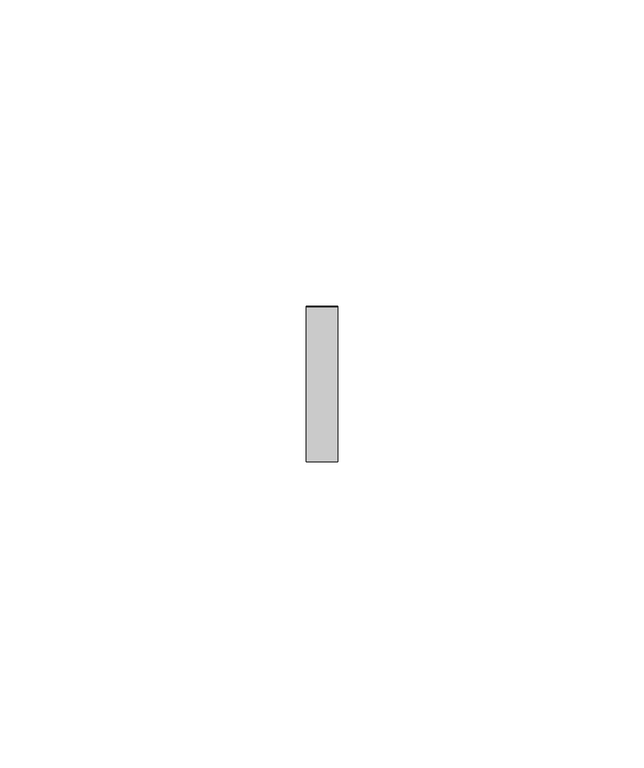
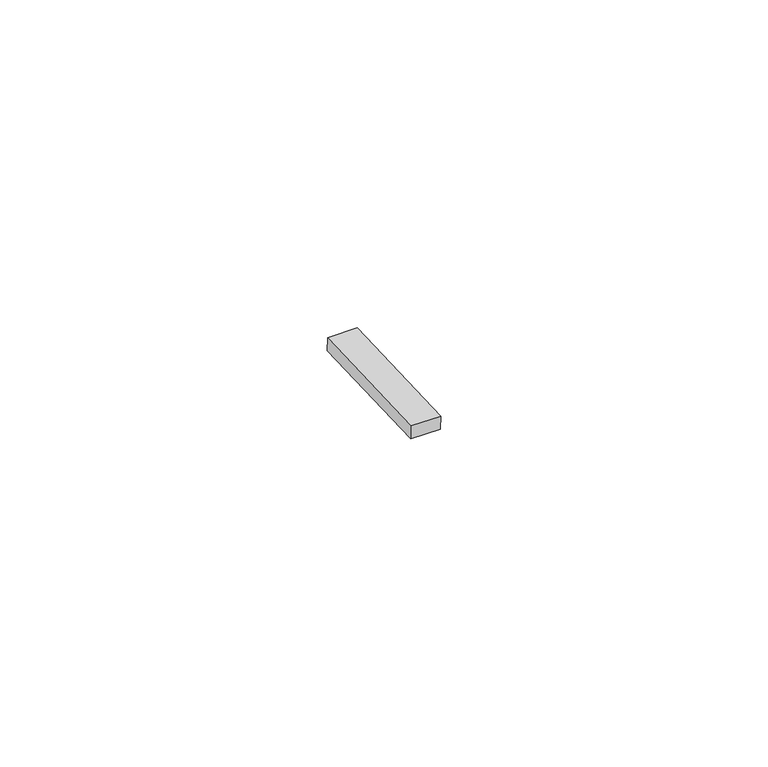
"""IFC4 building model written with IfcOpenShell, lengths in millimetres: proxy geometry, Inner panel:Inner panel:1:Inner panel:1 : Inner panel:Inner panel:300324:2:Inner panel:1:Inner panel:1 : Inner panel:Inner panel:300324:2 : Inner panel:Inner panel:1:Inner panel:1 : Inner panel:Inner panel:300324:300043:111 : Inner panel:Inner panel:1:Inner panel:1 : Inner panel:Inner panel:300324:2:Inner panel:1:Inner panel:1 : Inner panel:Inner panel:300324:2 : Inner panel:Inner panel:1:Inner panel:1 : Inner panel:Inner panel:300324:300043:308120."""

from ifc_helpers import new_model, si_unit, frame, origin, place, context, project, spatial, polyline, outline, extrude, source, transform, mapped, element, save


def generic_models_45de1fa8(model_context):
    return source(origin(), model_context, "Body", "SweptSolid", [
        extrude(outline(polyline([(0.0, -25.3999999), (0.0, 0.0), (5.2138089, 0.0), (5.2138089, -25.3999999), (0.0, -25.3999999)])), frame((593530.195117, -568962.1117339, 8771.3846899), z_axis=(0.0, -0.041630544712223896, 0.9991330730923502), x_axis=(-1.0, 0.0, 0.0)), (0.0, 0.0, 1.0), 2.4763745),
    ])


if __name__ == "__main__":
    model = new_model("IFC4")
    model_context = context("Model", 3, world=origin())
    ifc_project = project(units=[si_unit("LENGTHUNIT", "METRE", prefix="MILLI")], contexts=[model_context])
    site = spatial("IfcSite", under=ifc_project)
    building = spatial("IfcBuilding", under=site)
    placement = place(None, origin())
    generic_models_shape = generic_models_45de1fa8(model_context)
    element("IfcBuildingElementProxy", 1, Name="Inner panel:Inner panel:1:Inner panel:1 : Inner panel:Inner panel:300324:2:Inner panel:1:Inner panel:1 : Inner panel:Inner panel:300324:2 : Inner panel:Inner panel:1:Inner panel:1 : Inner panel:Inner panel:300324:300043:111 : Inner panel:Inner panel:1:Inner panel:1 : Inner panel:Inner panel:300324:2:Inner panel:1:Inner panel:1 : Inner panel:Inner panel:300324:2 : Inner panel:Inner panel:1:Inner panel:1 : Inner panel:Inner panel:300324:300043:308120", ObjectType="Inner panel:Inner panel:1:Inner panel:1 : Inner panel:Inner panel:300324:2:Inner panel:1:Inner panel:1 : Inner panel:Inner panel:300324:2 : Inner panel:Inner panel:1:Inner panel:1 : Inner panel:Inner panel:300324:300043:111 : Inner panel:Inner panel:1:Inner panel:1 : Inner panel:Inner panel:300324:2:Inner panel:1:Inner panel:1 : Inner panel:Inner panel:300324:2 : Inner panel:Inner panel:1:Inner panel:1 : Inner panel:Inner panel:300324:300043:308120", at=placement, inside=building, context=model_context, shape_type="MappedRepresentation", body=[
        mapped(generic_models_shape, transform((0.0, 0.0, 0.0), x_axis=(1.0, 0.0, 0.0), y_axis=(0.0, 1.0, 0.0), z_axis=(0.0, 0.0, 1.0))),
    ])
    save(model, "model.ifc")

# Revit data of these elements
# Type "Inner panel:Inner panel:1:Inner panel:1 : Inner panel:Inner panel:300324:2:Inner panel:1:Inner panel:1 : Inner panel:Inner panel:300324:2 : Inner panel:Inner panel:1:Inner panel:1 : Inner panel:Inner panel:300324:300043:111 : Inner panel:Inner panel:1:Inner panel:1 : Inner panel:Inner panel:300324:2:Inner panel:1:Inner panel:1 : Inner panel:Inner panel:300324:2 : Inner panel:Inner panel:1:Inner panel:1 : Inner panel:Inner panel:300324:300043:308120"
#   NameOverride = "Inner panel:Inner panel:1:Inner panel:1 : Inner panel:Inner panel:300324:2:Inner panel:1:Inner panel:1 : Inner panel:Inner panel:300324:2 : Inner panel:Inner panel:1:Inner panel:1 : Inner panel:Inner panel:300324:300043:308120"
#   ObjectTypeOverride = "Inner panel:1:Inner panel:1 : Inner panel:Inner panel:300324:2 : Inner panel:Inner panel:1:Inner panel:1 : Inner panel:Inner panel:300324:300043"
#   Reference = "Inner panel"
#   Tag = "308120"
# Element 1 (IfcBuildingElementProxy, "Inner panel:Inner panel:1:Inner panel:1 : Inner panel:Inner panel:300324:2:Inner panel:1:Inner panel:1 : Inner panel:Inner panel:300324:2 : Inner panel:Inner panel:1:Inner panel:1 : Inner panel:Inner panel:300324:300043:111 : Inner panel:Inner panel:1:Inner panel:1 : Inner panel:Inner panel:300324:2:Inner panel:1:Inner panel:1 : Inner panel:Inner panel:300324:2 : Inner panel:Inner panel:1:Inner panel:1 : Inner panel:Inner panel:300324:300043:308120")
#   Materials on its faces: "AT CLIP - 1\" WIDE NON ABSORBENT, WEATHER-RESISTANT NEOPRENE/EPDM/SBR FOAM"
# Materials
#   "AT CLIP - 1\" WIDE NON ABSORBENT, WEATHER-RESISTANT NEOPRENE/EPDM/SBR FOAM": class "Generic", colour RGB 85 85 85, transparency 0, Cost = 0
